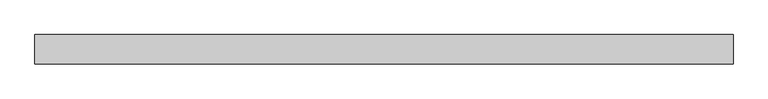
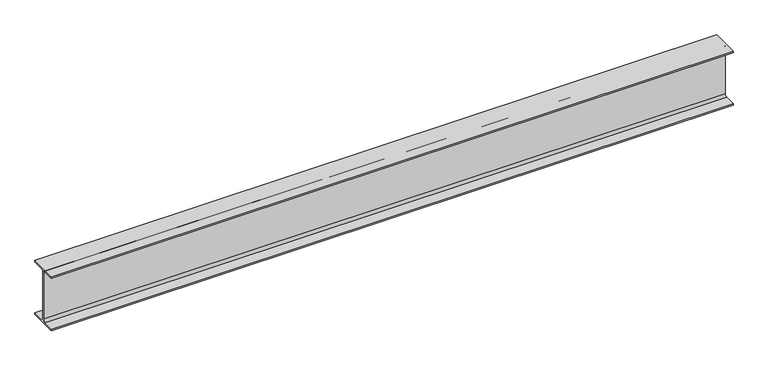
"""IFC4 building model written with IfcOpenShell, lengths in millimetres: beam geometry, 0912_Steel Framing_H-KSD3502 : H_SB_AR_S02_H-300x150x6.5x9_Stair."""

from ifc_helpers import new_model, si_unit, point, frame, frame_2d, origin, place, context, project, spatial, polyline, circle_curve, trimmed, segment, composite_curve, outline, extrude, source, transform, mapped, element, save


def beam_d6c2ad6f(model_context):
    return source(origin(), model_context, "Body", "SweptSolid", [
        extrude(outline(composite_curve([segment(polyline([(75.0, -141.0), (75.0, -150.0), (-75.0, -150.0), (-75.0, -141.0), (-16.25, -141.0)]), True, "CONTINUOUS"), segment(trimmed(circle_curve(frame_2d((-16.25, -128.0)), 13.0), [point((-16.25, -141.0))], [point((-3.25, -128.0))], True, "CARTESIAN"), True, "CONTINUOUS"), segment(polyline([(-3.25, -128.0), (-3.25, 128.0)]), True, "CONTINUOUS"), segment(trimmed(circle_curve(frame_2d((-16.25, 128.0)), 13.0), [point((-3.25, 128.0))], [point((-16.25, 141.0))], True, "CARTESIAN"), True, "CONTINUOUS"), segment(polyline([(-16.25, 141.0), (-75.0, 141.0), (-75.0, 150.0), (75.0, 150.0), (75.0, 141.0), (16.25, 141.0)]), True, "CONTINUOUS"), segment(trimmed(circle_curve(frame_2d((16.25, 128.0)), 13.0), [point((16.25, 141.0))], [point((3.25, 128.0))], True, "CARTESIAN"), True, "CONTINUOUS"), segment(polyline([(3.25, 128.0), (3.25, -128.0)]), True, "CONTINUOUS"), segment(trimmed(circle_curve(frame_2d((16.25, -128.0)), 13.0), [point((3.25, -128.0))], [point((16.25, -141.0))], True, "CARTESIAN"), True, "CONTINUOUS"), segment(polyline([(16.25, -141.0), (75.0, -141.0)]), True, "CONTINUOUS")], self_intersect=False)), frame((-1762.4373575, 0.0, 0.0), z_axis=(1.0, 0.0, 0.0), x_axis=(0.0, 1.0, 0.0)), (0.0, 0.0, 1.0), 3574.3249285),
    ])


if __name__ == "__main__":
    model = new_model("IFC4")
    model_context = context("Model", 3, world=origin())
    ifc_project = project(units=[si_unit("LENGTHUNIT", "METRE", prefix="MILLI")], contexts=[model_context])
    site = spatial("IfcSite", under=ifc_project)
    building = spatial("IfcBuilding", under=site)
    placement = place(None, origin())
    beam_shape = beam_d6c2ad6f(model_context)
    element("IfcBeam", 1, ObjectType="0912_Steel Framing_H-KSD3502 : H_SB_AR_S02_H-300x150x6.5x9_Stair", at=placement, inside=building, context=model_context, shape_type="MappedRepresentation", body=[
        mapped(beam_shape, transform((0.0, 0.0, 0.0), x_axis=(1.0, 0.0, 0.0), y_axis=(0.0, 1.0, 0.0), z_axis=(0.0, 0.0, 1.0))),
    ])
    save(model, "model.ifc")

# Revit data of these elements
# Type "0912_Steel Framing_H-KSD3502 : H_SB_AR_S02_H-300x150x6.5x9_Stair"
#   H_Q'ty Cal Type Tag = "SB-Q2"
#   H_WM Code_1 = "S01AA073-00001 |  | TON | Main Steel Structure Fabrication Work | Shelter/Building | Medium Steel - Standard |  |  |  |  |  |  | Material: (   ) | (90)KG/M>Weight≥(30)KG/M | S01AA073-00001 Main Steel Structure Fabrication Work Shelter/Building Medium Steel - Standard         | - Material: ( ASTM A36 )\n- (90)KG/M>Weight≥(30)KG/M"
#   H_WM Code_2 = "S03AA083-00001 |  | TON | Main Steel Structure Erection Work | Shelter/Building | Medium Steel |  |  |  |  |  |  | Material: (   ) | S03AA083-00001 Main Steel Structure Erection Work Shelter/Building Medium Steel         | - Material: ( ASTM A36 )"
#   H_WM Code_3 = "S01AA009-00001 |  | TON | Main Steel Structure Fabrication Work | Shelter/Building | Plates - Gusset, Stiffener, ETC | Material: (   ) | S01AA009-00001 Main Steel Structure Fabrication Work Shelter/Building Plates - Gusset, Stiffener, ETC         |"
#   H_WM Code_4 = "S41AA051-00001 |  | M2 | Steel Structure Paint Work | Shelter/Building | for Non-Fireproofed Steel Surface |  |  |  |  |  |  | Material: (   ) | S41AA051-00001 Steel Structure Paint Work Shelter/Building for Non-Fireproofed Steel Surface         |"
#   Width = 15.0 cm
#   Web Thickness = 0.65 cm
#   Web Fillet = 1.3 cm
#   Warping Constant = 107000.0 cm⁶
#   W = 0
#   Torsional Moment of Inertia = 9.9539 cm⁴
#   Section Area = 46.78 cm²
#   Plastic Modulus weak axis = 105.0 cm³
#   Plastic Modulus strong axis = 542.0 cm³
#   Perimeter = 1.17 m²/m
#   Nominal Weight = 36.70 kgf/m
#   Moment of Inertia weak axis = 508.00 cm⁴
#   Moment of Inertia strong axis = 7210.00 cm⁴
#   Height = 30.0 cm
#   Flange Thickness = 0.9 cm
#   Elastic Modulus weak axis = 67.7 cm³
#   Elastic Modulus strong axis = 481.0 cm³
#   Centroid Vertical = 15.0 cm
#   Centroid Horizontal = 7.5 cm
#   Ix = 72100000
#   Length [instance default] = 1524 mm
#   Zx = 542000
#   b = 150 mm
#   h = 300 mm
#   r = 13 mm
#   s = 6.5 mm
#   t = 9 mm
#   A = 0.004678 m²
#   Structural Material [instance default] = Steel, 45-345
#   Assembly Code = ""
# Element 1 (IfcBeam, "0912_Steel Framing_H-KSD3502 : H_SB_AR_S02_H-300x150x6.5x9_Stair")
#   Materials on its faces: "Steel, 45-345"
# Materials
#   "Steel, 45-345": class "Metal", colour RGB 189 187 185, transparency 0, Description = "Steel 345 MPa", Cost = 0
